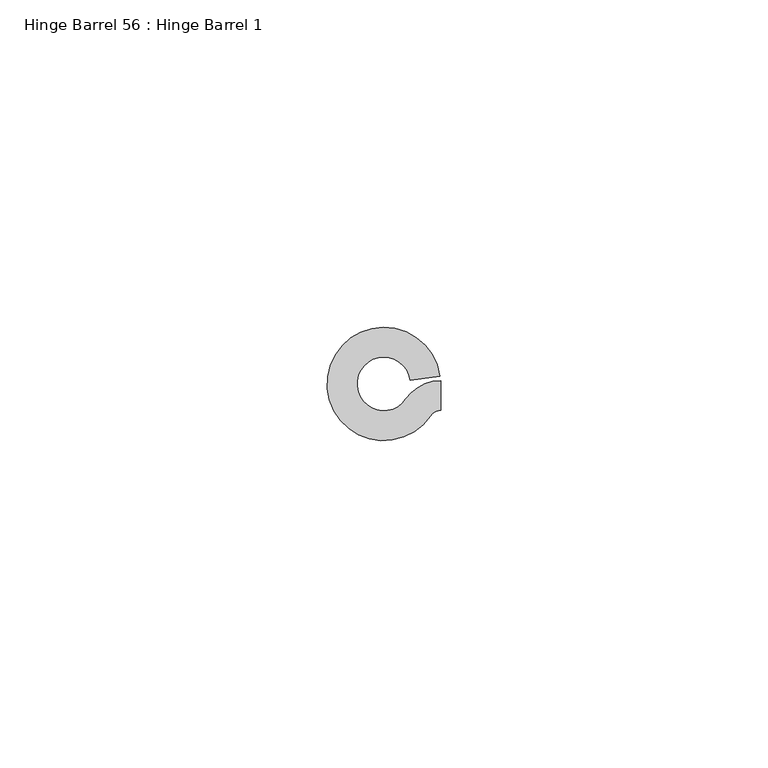
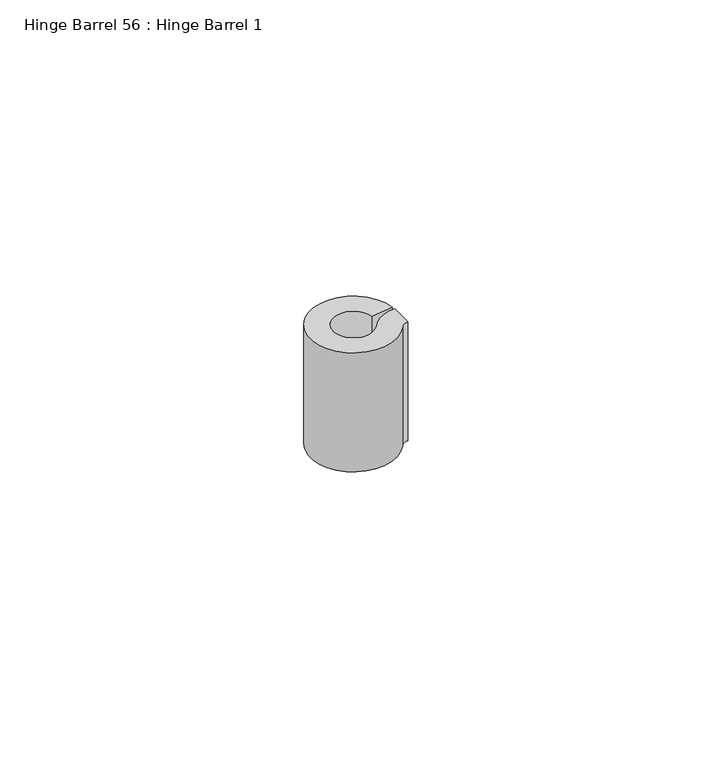
"""IFC4 building model written with IfcOpenShell, lengths in millimetres: proxy geometry, Hinge Barrel 56 : Hinge Barrel 1."""

from ifc_helpers import new_model, si_unit, point, frame, frame_2d, origin, place, context, project, spatial, polyline, circle_curve, trimmed, segment, composite_curve, outline, extrude, source, transform, mapped, element, save


def hinge_barrel_56_hinge_barrel_1_d11eb973(model_context):
    return source(origin(), model_context, "Body", "SweptSolid", [
        extrude(outline(composite_curve([segment(trimmed(circle_curve(frame_2d((587327.8245257, -536316.2443067)), 6.4044851), [point((587322.5194669, -536312.6563017))], [point((587327.8245257, -536309.8398216))], False, "CARTESIAN"), True, "CONTINUOUS"), segment(polyline([(587327.8245257, -536309.8398216), (587327.8245257, -536314.4038841)]), True, "CONTINUOUS"), segment(trimmed(circle_curve(frame_2d((587327.8245257, -536316.2443067)), 1.8404226), [point((587327.8245257, -536314.4038841))], [point((587326.3000393, -536315.2132409))], True, "CARTESIAN"), True, "CONTINUOUS"), segment(trimmed(circle_curve(frame_2d((587319.1320739, -536310.3652841)), 8.6534625), [point((587326.3000393, -536315.2132409))], [point((587327.7022899, -536309.1678654))], False, "CARTESIAN"), True, "CONTINUOUS"), segment(polyline([(587327.7022899, -536309.1678654), (587323.1821338, -536309.7994153)]), True, "CONTINUOUS"), segment(trimmed(circle_curve(frame_2d((587319.1320739, -536310.3652841)), 4.0894), [point((587323.1821338, -536309.7994153))], [point((587322.5194669, -536312.6563017))], True, "CARTESIAN"), True, "CONTINUOUS")], self_intersect=False)), frame((0.0, 0.0, 336.55), z_axis=(0.0, 0.0, 1.0), x_axis=(1.0, 0.0, 0.0)), (0.0, 0.0, 1.0), 25.4),
    ])


if __name__ == "__main__":
    model = new_model("IFC4")
    model_context = context("Model", 3, world=origin())
    ifc_project = project(units=[si_unit("LENGTHUNIT", "METRE", prefix="MILLI")], contexts=[model_context])
    site = spatial("IfcSite", under=ifc_project)
    building = spatial("IfcBuilding", under=site)
    placement = place(None, origin())
    hinge_barrel_56_hinge_barrel_1_shape = hinge_barrel_56_hinge_barrel_1_d11eb973(model_context)
    element("IfcBuildingElementProxy", 1, Name="Hinge Barrel 56 : Hinge Barrel 1", ObjectType="Hinge Barrel 56 : Hinge Barrel 1", at=placement, inside=building, context=model_context, shape_type="MappedRepresentation", body=[
        mapped(hinge_barrel_56_hinge_barrel_1_shape, transform((0.0, 0.0, 0.0), x_axis=(1.0, 0.0, 0.0), y_axis=(0.0, 1.0, 0.0), z_axis=(0.0, 0.0, 1.0))),
    ])
    save(model, "model.ifc")

# Revit data of these elements
# Element 1 (IfcBuildingElementProxy, "Hinge Barrel 56 : Hinge Barrel 1")
#   Materials on its faces: "6\"X6\" WELD-ON STL BUTT HINGE"
# Materials
#   "6\"X6\" WELD-ON STL BUTT HINGE": class "Metal", colour RGB 189 187 185, transparency 0, Description = "Carbon steel", Cost = 0
